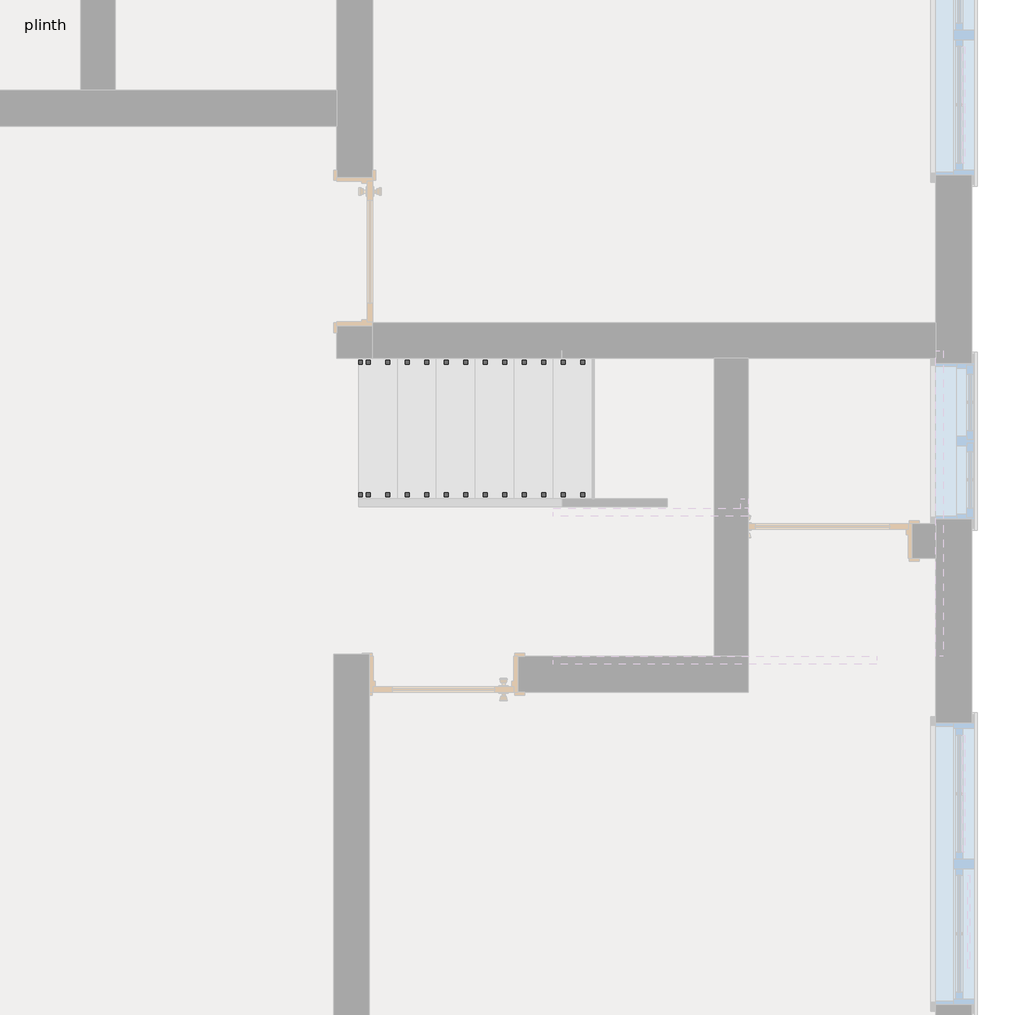
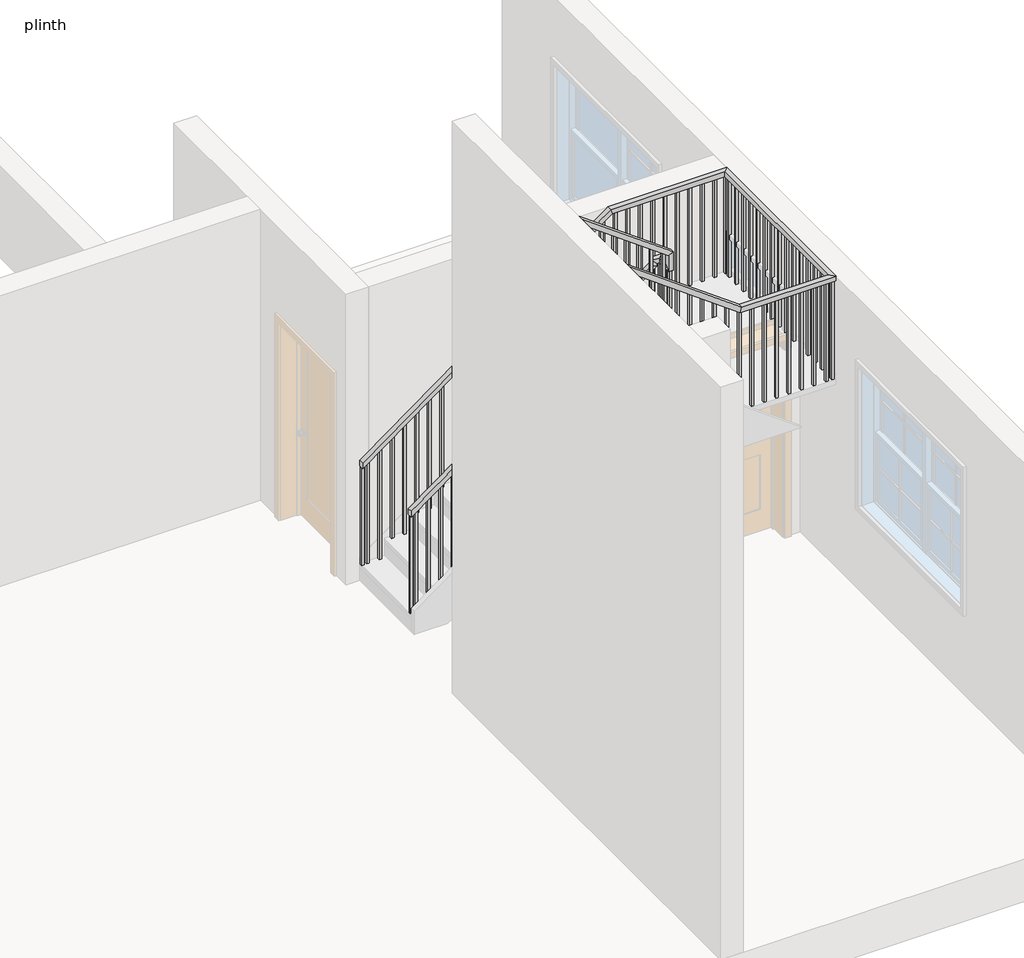
# One storey, part 2 of 3: 2 railings.
"""IFC4 building model written with IfcOpenShell, lengths in millimetres."""

from ifc_helpers import new_model, si_unit, frame, origin, place, context, project, spatial, polyline, outline, extrude, faceted_brep, element, save

model = new_model("IFC4")

# Units and contexts
model_context = context("Model", 3, world=origin())
ifc_project = project(units=[si_unit("LENGTHUNIT", "METRE", prefix="MILLI")], contexts=[model_context])

# Site, building, storey
site = spatial("IfcSite", under=ifc_project)
building = spatial("IfcBuilding", under=site)
storey = spatial("IfcBuildingStorey", under=building, Name="plinth", Elevation=450.0)

# Railings
placement = place(None, origin())
element("IfcRailing", 1, ObjectType="1100mm", at=placement, inside=storey, context=model_context, shape_type="SolidModel", body=[
    faceted_brep([(-8719.2253352, 6758.6914588, 1732.3529412), (-8719.2253352, 6758.6914588, 1670.4651087), (-8719.2253352, 6708.6914588, 1670.4651087), (-8719.2253352, 6708.6914588, 1732.3529412), (-6293.8253352, 6758.6914588, 3501.4682353), (-6243.8253352, 6758.6914588, 3476.0509911), (-6243.8253352, 6708.6914588, 3476.0509911), (-6293.8253352, 6708.6914588, 3501.4682353), (-6293.8253352, 6758.6914588, 3555.8823529), (-6243.8253352, 6758.6914588, 3505.8823529), (-6243.8253352, 6708.6914588, 3505.8823529), (-6293.8253352, 6708.6914588, 3555.8823529), (-6168.8253352, 6758.6914588, 3555.8823529), (-6168.8253352, 6758.6914588, 3505.8823529), (-6218.8253352, 6708.6914588, 3505.8823529), (-6218.8253352, 6708.6914588, 3555.8823529), (-6168.8253352, 6633.6914588, 3555.8823529), (-6168.8253352, 6633.6914588, 3505.8823529), (-6218.8253352, 6633.6914588, 3505.8823529), (-6218.8253352, 6633.6914588, 3555.8823529), (-6168.8253352, 6597.8914588, 3555.8823529), (-6218.8253352, 6597.8914588, 3555.8823529), (-6218.8253352, 6547.8914588, 3505.8823529), (-6168.8253352, 6547.8914588, 3505.8823529)], [[[0, 1, 2, 3]], [[1, 0, 4, 5]], [[2, 1, 5, 6]], [[3, 2, 6, 7]], [[0, 3, 7, 4]], [[5, 4, 8, 9]], [[6, 5, 9, 10]], [[7, 6, 10, 11]], [[4, 7, 11, 8]], [[9, 8, 12, 13]], [[10, 9, 13, 14]], [[11, 10, 14, 15]], [[8, 11, 15, 12]], [[13, 12, 16, 17]], [[14, 13, 17, 18]], [[15, 14, 18, 19]], [[12, 15, 19, 16]], [[20, 21, 22, 23]], [[17, 16, 20, 23]], [[18, 17, 23, 22]], [[19, 18, 22, 21]], [[16, 19, 21, 20]]]),
    faceted_brep([(-6168.8253352, 6597.8914588, 3555.8823529), (-6168.8253352, 6547.8914588, 3505.8823529), (-6218.8253352, 6547.8914588, 3505.8823529), (-6218.8253352, 6597.8914588, 3555.8823529), (-6168.8253352, 6597.8914588, 3701.4729412), (-6218.8253352, 6597.8914588, 3676.055697), (-6218.8253352, 6547.8914588, 3676.055697), (-6168.8253352, 6547.8914588, 3701.4729412)], [[[0, 1, 2, 3]], [[4, 5, 6, 7]], [[1, 0, 4, 7]], [[2, 1, 7, 6]], [[3, 2, 6, 5]], [[0, 3, 5, 4]]]),
    faceted_brep([(-6168.8253352, 6547.8914588, 3701.4729412), (-6218.8253352, 6547.8914588, 3676.055697), (-6218.8253352, 6597.8914588, 3676.055697), (-6168.8253352, 6597.8914588, 3701.4729412), (-7469.2253352, 6547.8914588, 4650.0), (-7469.2253352, 6597.8914588, 4650.0), (-7469.2253352, 6597.8914588, 4588.1121675), (-7469.2253352, 6547.8914588, 4588.1121675)], [[[0, 1, 2, 3]], [[4, 5, 6, 7]], [[1, 0, 4, 7]], [[2, 1, 7, 6]], [[3, 2, 6, 5]], [[0, 3, 5, 4]]]),
    extrude(outline(polyline([(3367.6470588, -7368.8253352), (4514.8792264, -7368.8253352), (4533.1145205, -7393.8253352), (3367.6470588, -7393.8253352), (3367.6470588, -7368.8253352)])), frame((0.0, 6560.3914588, 0.0), z_axis=(0.0, 1.0, 0.0), x_axis=(0.0, 0.0, 1.0)), (0.0, 0.0, 1.0), 25.0),
    extrude(outline(polyline([(3367.6470588, -7243.8253352), (4423.7027558, -7243.8253352), (4441.9380499, -7268.8253352), (3367.6470588, -7268.8253352), (3367.6470588, -7243.8253352)])), frame((0.0, 6560.3914588, 0.0), z_axis=(0.0, 1.0, 0.0), x_axis=(0.0, 0.0, 1.0)), (0.0, 0.0, 1.0), 25.0),
    extrude(outline(polyline([(3185.2941176, -7118.8253352), (4332.5262852, -7118.8253352), (4350.7615793, -7143.8253352), (3185.2941176, -7143.8253352), (3185.2941176, -7118.8253352)])), frame((0.0, 6560.3914588, 0.0), z_axis=(0.0, 1.0, 0.0), x_axis=(0.0, 0.0, 1.0)), (0.0, 0.0, 1.0), 25.0),
    extrude(outline(polyline([(3185.2941176, -6993.8253352), (4241.3498146, -6993.8253352), (4259.5851087, -7018.8253352), (3185.2941176, -7018.8253352), (3185.2941176, -6993.8253352)])), frame((0.0, 6560.3914588, 0.0), z_axis=(0.0, 1.0, 0.0), x_axis=(0.0, 0.0, 1.0)), (0.0, 0.0, 1.0), 25.0),
    extrude(outline(polyline([(3002.9411765, -6868.8253352), (4150.173344, -6868.8253352), (4168.4086381, -6893.8253352), (3002.9411765, -6893.8253352), (3002.9411765, -6868.8253352)])), frame((0.0, 6560.3914588, 0.0), z_axis=(0.0, 1.0, 0.0), x_axis=(0.0, 0.0, 1.0)), (0.0, 0.0, 1.0), 25.0),
    extrude(outline(polyline([(3002.9411765, -6743.8253352), (4058.9968734, -6743.8253352), (4077.2321675, -6768.8253352), (3002.9411765, -6768.8253352), (3002.9411765, -6743.8253352)])), frame((0.0, 6560.3914588, 0.0), z_axis=(0.0, 1.0, 0.0), x_axis=(0.0, 0.0, 1.0)), (0.0, 0.0, 1.0), 25.0),
    extrude(outline(polyline([(2820.5882353, -6618.8253352), (3967.8204028, -6618.8253352), (3986.055697, -6643.8253352), (2820.5882353, -6643.8253352), (2820.5882353, -6618.8253352)])), frame((0.0, 6560.3914588, 0.0), z_axis=(0.0, 1.0, 0.0), x_axis=(0.0, 0.0, 1.0)), (0.0, 0.0, 1.0), 25.0),
    extrude(outline(polyline([(2820.5882353, -6493.8253352), (3876.6439322, -6493.8253352), (3894.8792264, -6518.8253352), (2820.5882353, -6518.8253352), (2820.5882353, -6493.8253352)])), frame((0.0, 6560.3914588, 0.0), z_axis=(0.0, 1.0, 0.0), x_axis=(0.0, 0.0, 1.0)), (0.0, 0.0, 1.0), 25.0),
    extrude(outline(polyline([(2638.2352941, -6368.8253352), (3785.4674617, -6368.8253352), (3803.7027558, -6393.8253352), (2638.2352941, -6393.8253352), (2638.2352941, -6368.8253352)])), frame((0.0, 6560.3914588, 0.0), z_axis=(0.0, 1.0, 0.0), x_axis=(0.0, 0.0, 1.0)), (0.0, 0.0, 1.0), 25.0),
    extrude(outline(polyline([(2638.2352941, -6243.8253352), (3694.2909911, -6243.8253352), (3712.5262852, -6268.8253352), (2638.2352941, -6268.8253352), (2638.2352941, -6243.8253352)])), frame((0.0, 6560.3914588, 0.0), z_axis=(0.0, 1.0, 0.0), x_axis=(0.0, 0.0, 1.0)), (0.0, 0.0, 1.0), 25.0),
    extrude(outline(polyline([(-6206.3253352, 6683.6914588), (-6181.3253352, 6683.6914588), (-6181.3253352, 6658.6914588), (-6206.3253352, 6658.6914588), (-6206.3253352, 6683.6914588)])), frame((0.0, 0.0, 2455.8823529), z_axis=(0.0, 0.0, 1.0), x_axis=(1.0, 0.0, 0.0)), (0.0, 0.0, 1.0), 1050.0),
    extrude(outline(polyline([(-6294.2253352, 6721.1914588), (-6294.2253352, 6746.1914588), (-6269.2253352, 6746.1914588), (-6269.2253352, 6721.1914588), (-6294.2253352, 6721.1914588)])), frame((0.0, 0.0, 2273.5294118), z_axis=(0.0, 0.0, 1.0), x_axis=(1.0, 0.0, 0.0)), (0.0, 0.0, 1.0), 1232.3529412),
    extrude(outline(polyline([(3348.1121675, -6419.2253352), (2273.5294118, -6419.2253352), (2273.5294118, -6394.2253352), (3366.3474617, -6394.2253352), (3348.1121675, -6419.2253352)])), frame((0.0, 6721.1914588, 0.0), z_axis=(0.0, 1.0, 0.0), x_axis=(0.0, 0.0, 1.0)), (0.0, 0.0, 1.0), 25.0),
    extrude(outline(polyline([(3256.935697, -6544.2253352), (2091.1764706, -6544.2253352), (2091.1764706, -6519.2253352), (3275.1709911, -6519.2253352), (3256.935697, -6544.2253352)])), frame((0.0, 6721.1914588, 0.0), z_axis=(0.0, 1.0, 0.0), x_axis=(0.0, 0.0, 1.0)), (0.0, 0.0, 1.0), 25.0),
    extrude(outline(polyline([(3165.7592264, -6669.2253352), (2091.1764706, -6669.2253352), (2091.1764706, -6644.2253352), (3183.9945205, -6644.2253352), (3165.7592264, -6669.2253352)])), frame((0.0, 6721.1914588, 0.0), z_axis=(0.0, 1.0, 0.0), x_axis=(0.0, 0.0, 1.0)), (0.0, 0.0, 1.0), 25.0),
    extrude(outline(polyline([(3074.5827558, -6794.2253352), (1908.8235294, -6794.2253352), (1908.8235294, -6769.2253352), (3092.8180499, -6769.2253352), (3074.5827558, -6794.2253352)])), frame((0.0, 6721.1914588, 0.0), z_axis=(0.0, 1.0, 0.0), x_axis=(0.0, 0.0, 1.0)), (0.0, 0.0, 1.0), 25.0),
    extrude(outline(polyline([(2983.4062852, -6919.2253352), (1908.8235294, -6919.2253352), (1908.8235294, -6894.2253352), (3001.6415793, -6894.2253352), (2983.4062852, -6919.2253352)])), frame((0.0, 6721.1914588, 0.0), z_axis=(0.0, 1.0, 0.0), x_axis=(0.0, 0.0, 1.0)), (0.0, 0.0, 1.0), 25.0),
    extrude(outline(polyline([(2892.2298146, -7044.2253352), (1726.4705882, -7044.2253352), (1726.4705882, -7019.2253352), (2910.4651087, -7019.2253352), (2892.2298146, -7044.2253352)])), frame((0.0, 6721.1914588, 0.0), z_axis=(0.0, 1.0, 0.0), x_axis=(0.0, 0.0, 1.0)), (0.0, 0.0, 1.0), 25.0),
    extrude(outline(polyline([(2801.053344, -7169.2253352), (1726.4705882, -7169.2253352), (1726.4705882, -7144.2253352), (2819.2886381, -7144.2253352), (2801.053344, -7169.2253352)])), frame((0.0, 6721.1914588, 0.0), z_axis=(0.0, 1.0, 0.0), x_axis=(0.0, 0.0, 1.0)), (0.0, 0.0, 1.0), 25.0),
    extrude(outline(polyline([(2709.8768734, -7294.2253352), (1544.1176471, -7294.2253352), (1544.1176471, -7269.2253352), (2728.1121675, -7269.2253352), (2709.8768734, -7294.2253352)])), frame((0.0, 6721.1914588, 0.0), z_axis=(0.0, 1.0, 0.0), x_axis=(0.0, 0.0, 1.0)), (0.0, 0.0, 1.0), 25.0),
    extrude(outline(polyline([(2618.7004028, -7419.2253352), (1544.1176471, -7419.2253352), (1544.1176471, -7394.2253352), (2636.935697, -7394.2253352), (2618.7004028, -7419.2253352)])), frame((0.0, 6721.1914588, 0.0), z_axis=(0.0, 1.0, 0.0), x_axis=(0.0, 0.0, 1.0)), (0.0, 0.0, 1.0), 25.0),
    extrude(outline(polyline([(2527.5239322, -7544.2253352), (1361.7647059, -7544.2253352), (1361.7647059, -7519.2253352), (2545.7592264, -7519.2253352), (2527.5239322, -7544.2253352)])), frame((0.0, 6721.1914588, 0.0), z_axis=(0.0, 1.0, 0.0), x_axis=(0.0, 0.0, 1.0)), (0.0, 0.0, 1.0), 25.0),
    extrude(outline(polyline([(2436.3474617, -7669.2253352), (1361.7647059, -7669.2253352), (1361.7647059, -7644.2253352), (2454.5827558, -7644.2253352), (2436.3474617, -7669.2253352)])), frame((0.0, 6721.1914588, 0.0), z_axis=(0.0, 1.0, 0.0), x_axis=(0.0, 0.0, 1.0)), (0.0, 0.0, 1.0), 25.0),
    extrude(outline(polyline([(2345.1709911, -7794.2253352), (1179.4117647, -7794.2253352), (1179.4117647, -7769.2253352), (2363.4062852, -7769.2253352), (2345.1709911, -7794.2253352)])), frame((0.0, 6721.1914588, 0.0), z_axis=(0.0, 1.0, 0.0), x_axis=(0.0, 0.0, 1.0)), (0.0, 0.0, 1.0), 25.0),
    extrude(outline(polyline([(2253.9945205, -7919.2253352), (1179.4117647, -7919.2253352), (1179.4117647, -7894.2253352), (2272.2298146, -7894.2253352), (2253.9945205, -7919.2253352)])), frame((0.0, 6721.1914588, 0.0), z_axis=(0.0, 1.0, 0.0), x_axis=(0.0, 0.0, 1.0)), (0.0, 0.0, 1.0), 25.0),
    extrude(outline(polyline([(2162.8180499, -8044.2253352), (997.0588235, -8044.2253352), (997.0588235, -8019.2253352), (2181.053344, -8019.2253352), (2162.8180499, -8044.2253352)])), frame((0.0, 6721.1914588, 0.0), z_axis=(0.0, 1.0, 0.0), x_axis=(0.0, 0.0, 1.0)), (0.0, 0.0, 1.0), 25.0),
    extrude(outline(polyline([(2071.6415793, -8169.2253352), (997.0588235, -8169.2253352), (997.0588235, -8144.2253352), (2089.8768734, -8144.2253352), (2071.6415793, -8169.2253352)])), frame((0.0, 6721.1914588, 0.0), z_axis=(0.0, 1.0, 0.0), x_axis=(0.0, 0.0, 1.0)), (0.0, 0.0, 1.0), 25.0),
    extrude(outline(polyline([(1980.4651087, -8294.2253352), (814.7058824, -8294.2253352), (814.7058824, -8269.2253352), (1998.7004028, -8269.2253352), (1980.4651087, -8294.2253352)])), frame((0.0, 6721.1914588, 0.0), z_axis=(0.0, 1.0, 0.0), x_axis=(0.0, 0.0, 1.0)), (0.0, 0.0, 1.0), 25.0),
    extrude(outline(polyline([(1889.2886381, -8419.2253352), (814.7058824, -8419.2253352), (814.7058824, -8394.2253352), (1907.5239322, -8394.2253352), (1889.2886381, -8419.2253352)])), frame((0.0, 6721.1914588, 0.0), z_axis=(0.0, 1.0, 0.0), x_axis=(0.0, 0.0, 1.0)), (0.0, 0.0, 1.0), 25.0),
    extrude(outline(polyline([(1798.1121675, -8544.2253352), (632.3529412, -8544.2253352), (632.3529412, -8519.2253352), (1816.3474617, -8519.2253352), (1798.1121675, -8544.2253352)])), frame((0.0, 6721.1914588, 0.0), z_axis=(0.0, 1.0, 0.0), x_axis=(0.0, 0.0, 1.0)), (0.0, 0.0, 1.0), 25.0),
    extrude(outline(polyline([(1706.935697, -8669.2253352), (632.3529412, -8669.2253352), (632.3529412, -8644.2253352), (1725.1709911, -8644.2253352), (1706.935697, -8669.2253352)])), frame((0.0, 6721.1914588, 0.0), z_axis=(0.0, 1.0, 0.0), x_axis=(0.0, 0.0, 1.0)), (0.0, 0.0, 1.0), 25.0),
    extrude(outline(polyline([(-6206.3253352, 6585.3914588), (-6181.3253352, 6585.3914588), (-6181.3253352, 6560.3914588), (-6206.3253352, 6560.3914588), (-6206.3253352, 6585.3914588)])), frame((0.0, 0.0, 2455.8823529), z_axis=(0.0, 0.0, 1.0), x_axis=(1.0, 0.0, 0.0)), (0.0, 0.0, 1.0), 1050.0),
    extrude(outline(polyline([(-6206.3253352, 6721.1914588), (-6206.3253352, 6746.1914588), (-6181.3253352, 6746.1914588), (-6181.3253352, 6721.1914588), (-6206.3253352, 6721.1914588)])), frame((0.0, 0.0, 2455.8823529), z_axis=(0.0, 0.0, 1.0), x_axis=(1.0, 0.0, 0.0)), (0.0, 0.0, 1.0), 1050.0),
    extrude(outline(polyline([(3367.6470588, -7444.2253352), (4569.8768734, -7444.2253352), (4588.1121675, -7469.2253352), (3367.6470588, -7469.2253352), (3367.6470588, -7444.2253352)])), frame((0.0, 6560.3914588, 0.0), z_axis=(0.0, 1.0, 0.0), x_axis=(0.0, 0.0, 1.0)), (0.0, 0.0, 1.0), 25.0),
    extrude(outline(polyline([(1670.4651087, -8719.2253352), (632.3529412, -8719.2253352), (632.3529412, -8694.2253352), (1688.7004028, -8694.2253352), (1670.4651087, -8719.2253352)])), frame((0.0, 6721.1914588, 0.0), z_axis=(0.0, 1.0, 0.0), x_axis=(0.0, 0.0, 1.0)), (0.0, 0.0, 1.0), 25.0),
])
element("IfcRailing", 2, ObjectType="1100mm", at=placement, inside=storey, context=model_context, shape_type="SolidModel", body=[
    faceted_brep([(-8719.2253352, 7607.8914588, 1732.3529412), (-8719.2253352, 7607.8914588, 1670.4651087), (-8719.2253352, 7557.8914588, 1670.4651087), (-8719.2253352, 7557.8914588, 1732.3529412), (-6219.2253352, 7607.8914588, 3555.8823529), (-6202.9275004, 7607.8914588, 3505.8823529), (-6202.9275004, 7557.8914588, 3505.8823529), (-6219.2253352, 7557.8914588, 3555.8823529), (-5019.6253352, 7607.8914588, 3555.8823529), (-5019.6253352, 7607.8914588, 3505.8823529), (-5069.6253352, 7557.8914588, 3505.8823529), (-5069.6253352, 7557.8914588, 3555.8823529), (-5019.6253352, 5698.6914588, 3555.8823529), (-5019.6253352, 5698.6914588, 3505.8823529), (-5069.6253352, 5748.6914588, 3505.8823529), (-5069.6253352, 5748.6914588, 3555.8823529), (-5969.2253352, 5698.6914588, 3555.8823529), (-5985.52317, 5698.6914588, 3505.8823529), (-5985.52317, 5748.6914588, 3505.8823529), (-5969.2253352, 5748.6914588, 3555.8823529), (-7469.2253352, 5698.6914588, 4650.0), (-7469.2253352, 5748.6914588, 4650.0), (-7469.2253352, 5748.6914588, 4588.1121675), (-7469.2253352, 5698.6914588, 4588.1121675)], [[[0, 1, 2, 3]], [[1, 0, 4, 5]], [[2, 1, 5, 6]], [[3, 2, 6, 7]], [[0, 3, 7, 4]], [[5, 4, 8, 9]], [[6, 5, 9, 10]], [[7, 6, 10, 11]], [[4, 7, 11, 8]], [[9, 8, 12, 13]], [[10, 9, 13, 14]], [[11, 10, 14, 15]], [[8, 11, 15, 12]], [[13, 12, 16, 17]], [[14, 13, 17, 18]], [[15, 14, 18, 19]], [[12, 15, 19, 16]], [[20, 21, 22, 23]], [[17, 16, 20, 23]], [[18, 17, 23, 22]], [[19, 18, 22, 21]], [[16, 19, 21, 20]]]),
    extrude(outline(polyline([(4497.2274617, -7344.6253352), (4515.4627558, -7369.6253352), (3367.6470588, -7369.6253352), (3367.6470588, -7344.6253352), (4497.2274617, -7344.6253352)])), frame((0.0, 5711.1914588, 0.0), z_axis=(0.0, 1.0, 0.0), x_axis=(0.0, 0.0, 1.0)), (0.0, 0.0, 1.0), 25.0),
    extrude(outline(polyline([(4406.0509911, -7219.6253352), (4424.2862852, -7244.6253352), (3367.6470588, -7244.6253352), (3367.6470588, -7219.6253352), (4406.0509911, -7219.6253352)])), frame((0.0, 5711.1914588, 0.0), z_axis=(0.0, 1.0, 0.0), x_axis=(0.0, 0.0, 1.0)), (0.0, 0.0, 1.0), 25.0),
    extrude(outline(polyline([(4314.8745205, -7094.6253352), (4333.1098146, -7119.6253352), (3185.2941176, -7119.6253352), (3185.2941176, -7094.6253352), (4314.8745205, -7094.6253352)])), frame((0.0, 5711.1914588, 0.0), z_axis=(0.0, 1.0, 0.0), x_axis=(0.0, 0.0, 1.0)), (0.0, 0.0, 1.0), 25.0),
    extrude(outline(polyline([(4223.6980499, -6969.6253352), (4241.933344, -6994.6253352), (3185.2941176, -6994.6253352), (3185.2941176, -6969.6253352), (4223.6980499, -6969.6253352)])), frame((0.0, 5711.1914588, 0.0), z_axis=(0.0, 1.0, 0.0), x_axis=(0.0, 0.0, 1.0)), (0.0, 0.0, 1.0), 25.0),
    extrude(outline(polyline([(4132.5215793, -6844.6253352), (4150.7568734, -6869.6253352), (3002.9411765, -6869.6253352), (3002.9411765, -6844.6253352), (4132.5215793, -6844.6253352)])), frame((0.0, 5711.1914588, 0.0), z_axis=(0.0, 1.0, 0.0), x_axis=(0.0, 0.0, 1.0)), (0.0, 0.0, 1.0), 25.0),
    extrude(outline(polyline([(4041.3451087, -6719.6253352), (4059.5804028, -6744.6253352), (3002.9411765, -6744.6253352), (3002.9411765, -6719.6253352), (4041.3451087, -6719.6253352)])), frame((0.0, 5711.1914588, 0.0), z_axis=(0.0, 1.0, 0.0), x_axis=(0.0, 0.0, 1.0)), (0.0, 0.0, 1.0), 25.0),
    extrude(outline(polyline([(3950.1686381, -6594.6253352), (3968.4039322, -6619.6253352), (2820.5882353, -6619.6253352), (2820.5882353, -6594.6253352), (3950.1686381, -6594.6253352)])), frame((0.0, 5711.1914588, 0.0), z_axis=(0.0, 1.0, 0.0), x_axis=(0.0, 0.0, 1.0)), (0.0, 0.0, 1.0), 25.0),
    extrude(outline(polyline([(3858.9921675, -6469.6253352), (3877.2274617, -6494.6253352), (2820.5882353, -6494.6253352), (2820.5882353, -6469.6253352), (3858.9921675, -6469.6253352)])), frame((0.0, 5711.1914588, 0.0), z_axis=(0.0, 1.0, 0.0), x_axis=(0.0, 0.0, 1.0)), (0.0, 0.0, 1.0), 25.0),
    extrude(outline(polyline([(3767.815697, -6344.6253352), (3786.0509911, -6369.6253352), (2638.2352941, -6369.6253352), (2638.2352941, -6344.6253352), (3767.815697, -6344.6253352)])), frame((0.0, 5711.1914588, 0.0), z_axis=(0.0, 1.0, 0.0), x_axis=(0.0, 0.0, 1.0)), (0.0, 0.0, 1.0), 25.0),
    extrude(outline(polyline([(3676.6392264, -6219.6253352), (3694.8745205, -6244.6253352), (2638.2352941, -6244.6253352), (2638.2352941, -6219.6253352), (3676.6392264, -6219.6253352)])), frame((0.0, 5711.1914588, 0.0), z_axis=(0.0, 1.0, 0.0), x_axis=(0.0, 0.0, 1.0)), (0.0, 0.0, 1.0), 25.0),
    extrude(outline(polyline([(3585.4627558, -6094.6253352), (3603.6980499, -6119.6253352), (2455.8823529, -6119.6253352), (2455.8823529, -6094.6253352), (3585.4627558, -6094.6253352)])), frame((0.0, 5711.1914588, 0.0), z_axis=(0.0, 1.0, 0.0), x_axis=(0.0, 0.0, 1.0)), (0.0, 0.0, 1.0), 25.0),
    extrude(outline(polyline([(3494.2862852, -5969.6253352), (3512.5215793, -5994.6253352), (2455.8823529, -5994.6253352), (2455.8823529, -5969.6253352), (3494.2862852, -5969.6253352)])), frame((0.0, 5711.1914588, 0.0), z_axis=(0.0, 1.0, 0.0), x_axis=(0.0, 0.0, 1.0)), (0.0, 0.0, 1.0), 25.0),
    extrude(outline(polyline([(-5844.6253352, 5711.1914588), (-5869.6253352, 5711.1914588), (-5869.6253352, 5736.1914588), (-5844.6253352, 5736.1914588), (-5844.6253352, 5711.1914588)])), frame((0.0, 0.0, 2455.8823529), z_axis=(0.0, 0.0, 1.0), x_axis=(1.0, 0.0, 0.0)), (0.0, 0.0, 1.0), 1050.0),
    extrude(outline(polyline([(-5719.6253352, 5711.1914588), (-5744.6253352, 5711.1914588), (-5744.6253352, 5736.1914588), (-5719.6253352, 5736.1914588), (-5719.6253352, 5711.1914588)])), frame((0.0, 0.0, 2455.8823529), z_axis=(0.0, 0.0, 1.0), x_axis=(1.0, 0.0, 0.0)), (0.0, 0.0, 1.0), 1050.0),
    extrude(outline(polyline([(-5594.6253352, 5711.1914588), (-5619.6253352, 5711.1914588), (-5619.6253352, 5736.1914588), (-5594.6253352, 5736.1914588), (-5594.6253352, 5711.1914588)])), frame((0.0, 0.0, 2455.8823529), z_axis=(0.0, 0.0, 1.0), x_axis=(1.0, 0.0, 0.0)), (0.0, 0.0, 1.0), 1050.0),
    extrude(outline(polyline([(-5469.6253352, 5711.1914588), (-5494.6253352, 5711.1914588), (-5494.6253352, 5736.1914588), (-5469.6253352, 5736.1914588), (-5469.6253352, 5711.1914588)])), frame((0.0, 0.0, 2455.8823529), z_axis=(0.0, 0.0, 1.0), x_axis=(1.0, 0.0, 0.0)), (0.0, 0.0, 1.0), 1050.0),
    extrude(outline(polyline([(-5344.6253352, 5711.1914588), (-5369.6253352, 5711.1914588), (-5369.6253352, 5736.1914588), (-5344.6253352, 5736.1914588), (-5344.6253352, 5711.1914588)])), frame((0.0, 0.0, 2455.8823529), z_axis=(0.0, 0.0, 1.0), x_axis=(1.0, 0.0, 0.0)), (0.0, 0.0, 1.0), 1050.0),
    extrude(outline(polyline([(-5219.6253352, 5711.1914588), (-5244.6253352, 5711.1914588), (-5244.6253352, 5736.1914588), (-5219.6253352, 5736.1914588), (-5219.6253352, 5711.1914588)])), frame((0.0, 0.0, 2455.8823529), z_axis=(0.0, 0.0, 1.0), x_axis=(1.0, 0.0, 0.0)), (0.0, 0.0, 1.0), 1050.0),
    extrude(outline(polyline([(-5094.6253352, 5711.1914588), (-5119.6253352, 5711.1914588), (-5119.6253352, 5736.1914588), (-5094.6253352, 5736.1914588), (-5094.6253352, 5711.1914588)])), frame((0.0, 0.0, 2455.8823529), z_axis=(0.0, 0.0, 1.0), x_axis=(1.0, 0.0, 0.0)), (0.0, 0.0, 1.0), 1050.0),
    extrude(outline(polyline([(-5032.1253352, 5782.8914588), (-5032.1253352, 5757.8914588), (-5057.1253352, 5757.8914588), (-5057.1253352, 5782.8914588), (-5032.1253352, 5782.8914588)])), frame((0.0, 0.0, 2455.8823529), z_axis=(0.0, 0.0, 1.0), x_axis=(1.0, 0.0, 0.0)), (0.0, 0.0, 1.0), 1050.0),
    extrude(outline(polyline([(-5032.1253352, 5907.8914588), (-5032.1253352, 5882.8914588), (-5057.1253352, 5882.8914588), (-5057.1253352, 5907.8914588), (-5032.1253352, 5907.8914588)])), frame((0.0, 0.0, 2455.8823529), z_axis=(0.0, 0.0, 1.0), x_axis=(1.0, 0.0, 0.0)), (0.0, 0.0, 1.0), 1050.0),
    extrude(outline(polyline([(-5032.1253352, 6032.8914588), (-5032.1253352, 6007.8914588), (-5057.1253352, 6007.8914588), (-5057.1253352, 6032.8914588), (-5032.1253352, 6032.8914588)])), frame((0.0, 0.0, 2455.8823529), z_axis=(0.0, 0.0, 1.0), x_axis=(1.0, 0.0, 0.0)), (0.0, 0.0, 1.0), 1050.0),
    extrude(outline(polyline([(-5032.1253352, 6157.8914588), (-5032.1253352, 6132.8914588), (-5057.1253352, 6132.8914588), (-5057.1253352, 6157.8914588), (-5032.1253352, 6157.8914588)])), frame((0.0, 0.0, 2455.8823529), z_axis=(0.0, 0.0, 1.0), x_axis=(1.0, 0.0, 0.0)), (0.0, 0.0, 1.0), 1050.0),
    extrude(outline(polyline([(-5032.1253352, 6282.8914588), (-5032.1253352, 6257.8914588), (-5057.1253352, 6257.8914588), (-5057.1253352, 6282.8914588), (-5032.1253352, 6282.8914588)])), frame((0.0, 0.0, 2455.8823529), z_axis=(0.0, 0.0, 1.0), x_axis=(1.0, 0.0, 0.0)), (0.0, 0.0, 1.0), 1050.0),
    extrude(outline(polyline([(-5032.1253352, 6407.8914588), (-5032.1253352, 6382.8914588), (-5057.1253352, 6382.8914588), (-5057.1253352, 6407.8914588), (-5032.1253352, 6407.8914588)])), frame((0.0, 0.0, 2455.8823529), z_axis=(0.0, 0.0, 1.0), x_axis=(1.0, 0.0, 0.0)), (0.0, 0.0, 1.0), 1050.0),
    extrude(outline(polyline([(-5032.1253352, 6532.8914588), (-5032.1253352, 6507.8914588), (-5057.1253352, 6507.8914588), (-5057.1253352, 6532.8914588), (-5032.1253352, 6532.8914588)])), frame((0.0, 0.0, 2455.8823529), z_axis=(0.0, 0.0, 1.0), x_axis=(1.0, 0.0, 0.0)), (0.0, 0.0, 1.0), 1050.0),
    extrude(outline(polyline([(-5032.1253352, 6657.8914588), (-5032.1253352, 6632.8914588), (-5057.1253352, 6632.8914588), (-5057.1253352, 6657.8914588), (-5032.1253352, 6657.8914588)])), frame((0.0, 0.0, 2455.8823529), z_axis=(0.0, 0.0, 1.0), x_axis=(1.0, 0.0, 0.0)), (0.0, 0.0, 1.0), 1050.0),
    extrude(outline(polyline([(-5032.1253352, 6782.8914588), (-5032.1253352, 6757.8914588), (-5057.1253352, 6757.8914588), (-5057.1253352, 6782.8914588), (-5032.1253352, 6782.8914588)])), frame((0.0, 0.0, 2455.8823529), z_axis=(0.0, 0.0, 1.0), x_axis=(1.0, 0.0, 0.0)), (0.0, 0.0, 1.0), 1050.0),
    extrude(outline(polyline([(-5032.1253352, 6907.8914588), (-5032.1253352, 6882.8914588), (-5057.1253352, 6882.8914588), (-5057.1253352, 6907.8914588), (-5032.1253352, 6907.8914588)])), frame((0.0, 0.0, 2455.8823529), z_axis=(0.0, 0.0, 1.0), x_axis=(1.0, 0.0, 0.0)), (0.0, 0.0, 1.0), 1050.0),
    extrude(outline(polyline([(-5032.1253352, 7032.8914588), (-5032.1253352, 7007.8914588), (-5057.1253352, 7007.8914588), (-5057.1253352, 7032.8914588), (-5032.1253352, 7032.8914588)])), frame((0.0, 0.0, 2455.8823529), z_axis=(0.0, 0.0, 1.0), x_axis=(1.0, 0.0, 0.0)), (0.0, 0.0, 1.0), 1050.0),
    extrude(outline(polyline([(-5032.1253352, 7157.8914588), (-5032.1253352, 7132.8914588), (-5057.1253352, 7132.8914588), (-5057.1253352, 7157.8914588), (-5032.1253352, 7157.8914588)])), frame((0.0, 0.0, 2455.8823529), z_axis=(0.0, 0.0, 1.0), x_axis=(1.0, 0.0, 0.0)), (0.0, 0.0, 1.0), 1050.0),
    extrude(outline(polyline([(-5032.1253352, 7282.8914588), (-5032.1253352, 7257.8914588), (-5057.1253352, 7257.8914588), (-5057.1253352, 7282.8914588), (-5032.1253352, 7282.8914588)])), frame((0.0, 0.0, 2455.8823529), z_axis=(0.0, 0.0, 1.0), x_axis=(1.0, 0.0, 0.0)), (0.0, 0.0, 1.0), 1050.0),
    extrude(outline(polyline([(-5032.1253352, 7407.8914588), (-5032.1253352, 7382.8914588), (-5057.1253352, 7382.8914588), (-5057.1253352, 7407.8914588), (-5032.1253352, 7407.8914588)])), frame((0.0, 0.0, 2455.8823529), z_axis=(0.0, 0.0, 1.0), x_axis=(1.0, 0.0, 0.0)), (0.0, 0.0, 1.0), 1050.0),
    extrude(outline(polyline([(-5032.1253352, 7532.8914588), (-5032.1253352, 7507.8914588), (-5057.1253352, 7507.8914588), (-5057.1253352, 7532.8914588), (-5032.1253352, 7532.8914588)])), frame((0.0, 0.0, 2455.8823529), z_axis=(0.0, 0.0, 1.0), x_axis=(1.0, 0.0, 0.0)), (0.0, 0.0, 1.0), 1050.0),
    extrude(outline(polyline([(-5169.2253352, 7595.3914588), (-5144.2253352, 7595.3914588), (-5144.2253352, 7570.3914588), (-5169.2253352, 7570.3914588), (-5169.2253352, 7595.3914588)])), frame((0.0, 0.0, 2455.8823529), z_axis=(0.0, 0.0, 1.0), x_axis=(1.0, 0.0, 0.0)), (0.0, 0.0, 1.0), 1050.0),
    extrude(outline(polyline([(-5294.2253352, 7595.3914588), (-5269.2253352, 7595.3914588), (-5269.2253352, 7570.3914588), (-5294.2253352, 7570.3914588), (-5294.2253352, 7595.3914588)])), frame((0.0, 0.0, 2455.8823529), z_axis=(0.0, 0.0, 1.0), x_axis=(1.0, 0.0, 0.0)), (0.0, 0.0, 1.0), 1050.0),
    extrude(outline(polyline([(-5419.2253352, 7595.3914588), (-5394.2253352, 7595.3914588), (-5394.2253352, 7570.3914588), (-5419.2253352, 7570.3914588), (-5419.2253352, 7595.3914588)])), frame((0.0, 0.0, 2455.8823529), z_axis=(0.0, 0.0, 1.0), x_axis=(1.0, 0.0, 0.0)), (0.0, 0.0, 1.0), 1050.0),
    extrude(outline(polyline([(-5544.2253352, 7595.3914588), (-5519.2253352, 7595.3914588), (-5519.2253352, 7570.3914588), (-5544.2253352, 7570.3914588), (-5544.2253352, 7595.3914588)])), frame((0.0, 0.0, 2455.8823529), z_axis=(0.0, 0.0, 1.0), x_axis=(1.0, 0.0, 0.0)), (0.0, 0.0, 1.0), 1050.0),
    extrude(outline(polyline([(-5669.2253352, 7595.3914588), (-5644.2253352, 7595.3914588), (-5644.2253352, 7570.3914588), (-5669.2253352, 7570.3914588), (-5669.2253352, 7595.3914588)])), frame((0.0, 0.0, 2455.8823529), z_axis=(0.0, 0.0, 1.0), x_axis=(1.0, 0.0, 0.0)), (0.0, 0.0, 1.0), 1050.0),
    extrude(outline(polyline([(-5794.2253352, 7595.3914588), (-5769.2253352, 7595.3914588), (-5769.2253352, 7570.3914588), (-5794.2253352, 7570.3914588), (-5794.2253352, 7595.3914588)])), frame((0.0, 0.0, 2455.8823529), z_axis=(0.0, 0.0, 1.0), x_axis=(1.0, 0.0, 0.0)), (0.0, 0.0, 1.0), 1050.0),
    extrude(outline(polyline([(-5919.2253352, 7595.3914588), (-5894.2253352, 7595.3914588), (-5894.2253352, 7570.3914588), (-5919.2253352, 7570.3914588), (-5919.2253352, 7595.3914588)])), frame((0.0, 0.0, 2455.8823529), z_axis=(0.0, 0.0, 1.0), x_axis=(1.0, 0.0, 0.0)), (0.0, 0.0, 1.0), 1050.0),
    extrude(outline(polyline([(-6044.2253352, 7595.3914588), (-6019.2253352, 7595.3914588), (-6019.2253352, 7570.3914588), (-6044.2253352, 7570.3914588), (-6044.2253352, 7595.3914588)])), frame((0.0, 0.0, 2455.8823529), z_axis=(0.0, 0.0, 1.0), x_axis=(1.0, 0.0, 0.0)), (0.0, 0.0, 1.0), 1050.0),
    extrude(outline(polyline([(-6169.2253352, 7595.3914588), (-6144.2253352, 7595.3914588), (-6144.2253352, 7570.3914588), (-6169.2253352, 7570.3914588), (-6169.2253352, 7595.3914588)])), frame((0.0, 0.0, 2455.8823529), z_axis=(0.0, 0.0, 1.0), x_axis=(1.0, 0.0, 0.0)), (0.0, 0.0, 1.0), 1050.0),
    extrude(outline(polyline([(2273.5294118, -6294.2253352), (2273.5294118, -6269.2253352), (3457.5239322, -6269.2253352), (3439.2886381, -6294.2253352), (2273.5294118, -6294.2253352)])), frame((0.0, 7570.3914588, 0.0), z_axis=(0.0, 1.0, 0.0), x_axis=(0.0, 0.0, 1.0)), (0.0, 0.0, 1.0), 25.0),
    extrude(outline(polyline([(2273.5294118, -6419.2253352), (2273.5294118, -6394.2253352), (3366.3474617, -6394.2253352), (3348.1121675, -6419.2253352), (2273.5294118, -6419.2253352)])), frame((0.0, 7570.3914588, 0.0), z_axis=(0.0, 1.0, 0.0), x_axis=(0.0, 0.0, 1.0)), (0.0, 0.0, 1.0), 25.0),
    extrude(outline(polyline([(2091.1764706, -6544.2253352), (2091.1764706, -6519.2253352), (3275.1709911, -6519.2253352), (3256.935697, -6544.2253352), (2091.1764706, -6544.2253352)])), frame((0.0, 7570.3914588, 0.0), z_axis=(0.0, 1.0, 0.0), x_axis=(0.0, 0.0, 1.0)), (0.0, 0.0, 1.0), 25.0),
    extrude(outline(polyline([(2091.1764706, -6669.2253352), (2091.1764706, -6644.2253352), (3183.9945205, -6644.2253352), (3165.7592264, -6669.2253352), (2091.1764706, -6669.2253352)])), frame((0.0, 7570.3914588, 0.0), z_axis=(0.0, 1.0, 0.0), x_axis=(0.0, 0.0, 1.0)), (0.0, 0.0, 1.0), 25.0),
    extrude(outline(polyline([(1908.8235294, -6794.2253352), (1908.8235294, -6769.2253352), (3092.8180499, -6769.2253352), (3074.5827558, -6794.2253352), (1908.8235294, -6794.2253352)])), frame((0.0, 7570.3914588, 0.0), z_axis=(0.0, 1.0, 0.0), x_axis=(0.0, 0.0, 1.0)), (0.0, 0.0, 1.0), 25.0),
    extrude(outline(polyline([(1908.8235294, -6919.2253352), (1908.8235294, -6894.2253352), (3001.6415793, -6894.2253352), (2983.4062852, -6919.2253352), (1908.8235294, -6919.2253352)])), frame((0.0, 7570.3914588, 0.0), z_axis=(0.0, 1.0, 0.0), x_axis=(0.0, 0.0, 1.0)), (0.0, 0.0, 1.0), 25.0),
    extrude(outline(polyline([(1726.4705882, -7044.2253352), (1726.4705882, -7019.2253352), (2910.4651087, -7019.2253352), (2892.2298146, -7044.2253352), (1726.4705882, -7044.2253352)])), frame((0.0, 7570.3914588, 0.0), z_axis=(0.0, 1.0, 0.0), x_axis=(0.0, 0.0, 1.0)), (0.0, 0.0, 1.0), 25.0),
    extrude(outline(polyline([(1726.4705882, -7169.2253352), (1726.4705882, -7144.2253352), (2819.2886381, -7144.2253352), (2801.053344, -7169.2253352), (1726.4705882, -7169.2253352)])), frame((0.0, 7570.3914588, 0.0), z_axis=(0.0, 1.0, 0.0), x_axis=(0.0, 0.0, 1.0)), (0.0, 0.0, 1.0), 25.0),
    extrude(outline(polyline([(1544.1176471, -7294.2253352), (1544.1176471, -7269.2253352), (2728.1121675, -7269.2253352), (2709.8768734, -7294.2253352), (1544.1176471, -7294.2253352)])), frame((0.0, 7570.3914588, 0.0), z_axis=(0.0, 1.0, 0.0), x_axis=(0.0, 0.0, 1.0)), (0.0, 0.0, 1.0), 25.0),
    extrude(outline(polyline([(1544.1176471, -7419.2253352), (1544.1176471, -7394.2253352), (2636.935697, -7394.2253352), (2618.7004028, -7419.2253352), (1544.1176471, -7419.2253352)])), frame((0.0, 7570.3914588, 0.0), z_axis=(0.0, 1.0, 0.0), x_axis=(0.0, 0.0, 1.0)), (0.0, 0.0, 1.0), 25.0),
    extrude(outline(polyline([(1361.7647059, -7544.2253352), (1361.7647059, -7519.2253352), (2545.7592264, -7519.2253352), (2527.5239322, -7544.2253352), (1361.7647059, -7544.2253352)])), frame((0.0, 7570.3914588, 0.0), z_axis=(0.0, 1.0, 0.0), x_axis=(0.0, 0.0, 1.0)), (0.0, 0.0, 1.0), 25.0),
    extrude(outline(polyline([(1361.7647059, -7669.2253352), (1361.7647059, -7644.2253352), (2454.5827558, -7644.2253352), (2436.3474617, -7669.2253352), (1361.7647059, -7669.2253352)])), frame((0.0, 7570.3914588, 0.0), z_axis=(0.0, 1.0, 0.0), x_axis=(0.0, 0.0, 1.0)), (0.0, 0.0, 1.0), 25.0),
    extrude(outline(polyline([(1179.4117647, -7794.2253352), (1179.4117647, -7769.2253352), (2363.4062852, -7769.2253352), (2345.1709911, -7794.2253352), (1179.4117647, -7794.2253352)])), frame((0.0, 7570.3914588, 0.0), z_axis=(0.0, 1.0, 0.0), x_axis=(0.0, 0.0, 1.0)), (0.0, 0.0, 1.0), 25.0),
    extrude(outline(polyline([(1179.4117647, -7919.2253352), (1179.4117647, -7894.2253352), (2272.2298146, -7894.2253352), (2253.9945205, -7919.2253352), (1179.4117647, -7919.2253352)])), frame((0.0, 7570.3914588, 0.0), z_axis=(0.0, 1.0, 0.0), x_axis=(0.0, 0.0, 1.0)), (0.0, 0.0, 1.0), 25.0),
    extrude(outline(polyline([(997.0588235, -8044.2253352), (997.0588235, -8019.2253352), (2181.053344, -8019.2253352), (2162.8180499, -8044.2253352), (997.0588235, -8044.2253352)])), frame((0.0, 7570.3914588, 0.0), z_axis=(0.0, 1.0, 0.0), x_axis=(0.0, 0.0, 1.0)), (0.0, 0.0, 1.0), 25.0),
    extrude(outline(polyline([(997.0588235, -8169.2253352), (997.0588235, -8144.2253352), (2089.8768734, -8144.2253352), (2071.6415793, -8169.2253352), (997.0588235, -8169.2253352)])), frame((0.0, 7570.3914588, 0.0), z_axis=(0.0, 1.0, 0.0), x_axis=(0.0, 0.0, 1.0)), (0.0, 0.0, 1.0), 25.0),
    extrude(outline(polyline([(814.7058824, -8294.2253352), (814.7058824, -8269.2253352), (1998.7004028, -8269.2253352), (1980.4651087, -8294.2253352), (814.7058824, -8294.2253352)])), frame((0.0, 7570.3914588, 0.0), z_axis=(0.0, 1.0, 0.0), x_axis=(0.0, 0.0, 1.0)), (0.0, 0.0, 1.0), 25.0),
    extrude(outline(polyline([(814.7058824, -8419.2253352), (814.7058824, -8394.2253352), (1907.5239322, -8394.2253352), (1889.2886381, -8419.2253352), (814.7058824, -8419.2253352)])), frame((0.0, 7570.3914588, 0.0), z_axis=(0.0, 1.0, 0.0), x_axis=(0.0, 0.0, 1.0)), (0.0, 0.0, 1.0), 25.0),
    extrude(outline(polyline([(632.3529412, -8544.2253352), (632.3529412, -8519.2253352), (1816.3474617, -8519.2253352), (1798.1121675, -8544.2253352), (632.3529412, -8544.2253352)])), frame((0.0, 7570.3914588, 0.0), z_axis=(0.0, 1.0, 0.0), x_axis=(0.0, 0.0, 1.0)), (0.0, 0.0, 1.0), 25.0),
    extrude(outline(polyline([(632.3529412, -8669.2253352), (632.3529412, -8644.2253352), (1725.1709911, -8644.2253352), (1706.935697, -8669.2253352), (632.3529412, -8669.2253352)])), frame((0.0, 7570.3914588, 0.0), z_axis=(0.0, 1.0, 0.0), x_axis=(0.0, 0.0, 1.0)), (0.0, 0.0, 1.0), 25.0),
    extrude(outline(polyline([(-5032.1253352, 5736.1914588), (-5032.1253352, 5711.1914588), (-5057.1253352, 5711.1914588), (-5057.1253352, 5736.1914588), (-5032.1253352, 5736.1914588)])), frame((0.0, 0.0, 2455.8823529), z_axis=(0.0, 0.0, 1.0), x_axis=(1.0, 0.0, 0.0)), (0.0, 0.0, 1.0), 1050.0),
    extrude(outline(polyline([(-5057.1253352, 7595.3914588), (-5032.1253352, 7595.3914588), (-5032.1253352, 7570.3914588), (-5057.1253352, 7570.3914588), (-5057.1253352, 7595.3914588)])), frame((0.0, 0.0, 2455.8823529), z_axis=(0.0, 0.0, 1.0), x_axis=(1.0, 0.0, 0.0)), (0.0, 0.0, 1.0), 1050.0),
    extrude(outline(polyline([(4569.8768734, -7444.2253352), (4588.1121675, -7469.2253352), (3367.6470588, -7469.2253352), (3367.6470588, -7444.2253352), (4569.8768734, -7444.2253352)])), frame((0.0, 5711.1914588, 0.0), z_axis=(0.0, 1.0, 0.0), x_axis=(0.0, 0.0, 1.0)), (0.0, 0.0, 1.0), 25.0),
    extrude(outline(polyline([(632.3529412, -8719.2253352), (632.3529412, -8694.2253352), (1688.7004028, -8694.2253352), (1670.4651087, -8719.2253352), (632.3529412, -8719.2253352)])), frame((0.0, 7570.3914588, 0.0), z_axis=(0.0, 1.0, 0.0), x_axis=(0.0, 0.0, 1.0)), (0.0, 0.0, 1.0), 25.0),
])

save(model, "model.ifc")

# Revit data of these elements
# Type "1100mm"
#   built-in parameter 1008612 = 0.019685 (stored number, unit not read)
#   built-in parameter 1008611 = 0.019685 (stored number, unit not read)
#   built-in parameter 1008609 = 0.902231 (stored number, unit not read)
#   built-in parameter 1008604 = 0.19685 (stored number, unit not read)
#   built-in parameter 1008603 = 0.164042 (stored number, unit not read)
#   Railing Height = 110 cm
#   built-in parameter 1008630 = 2
#   built-in parameter 1008610 = 2
#   built-in parameter 1008608 = 1
#   built-in parameter 1008618 = M_Baluster - Square : 25mm
# Elements 1, 2 (IfcRailing, "1100mm")
#   Phase Created = New Construction
